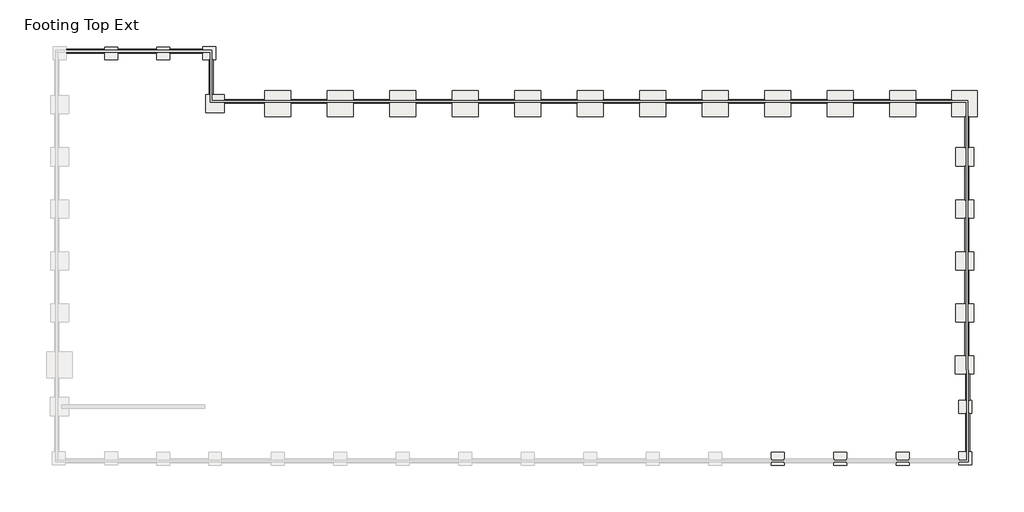
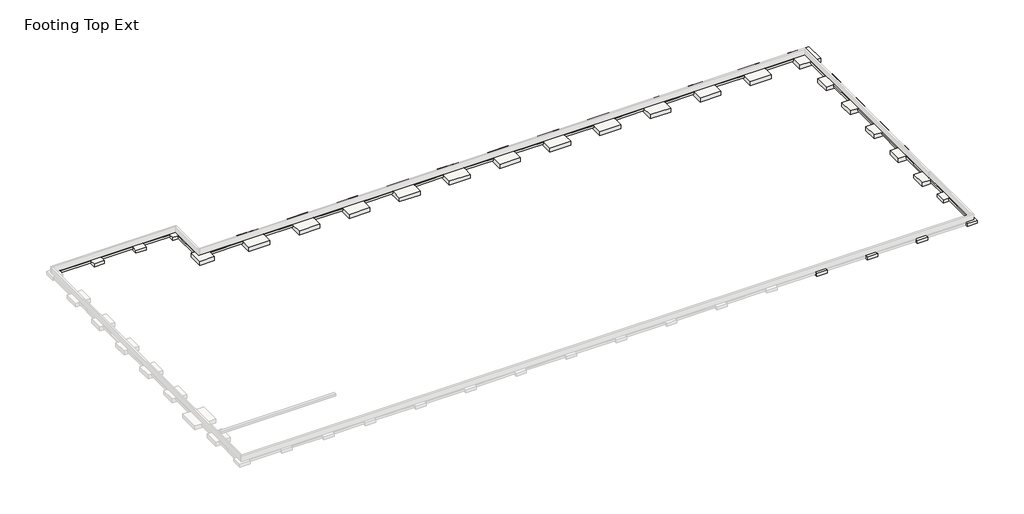
# One storey, part 2 of 2: 26 slabs, 5 footings.
"""IFC4 building model written with IfcOpenShell, lengths in millimetres."""

from ifc_helpers import new_model, si_unit, frame, origin, place, context, project, spatial, polyline, outline, extrude, faceted_brep, element, save

model = new_model("IFC4")

# Units and contexts
model_context = context("Model", 3, world=origin())
ifc_project = project(units=[si_unit("LENGTHUNIT", "METRE", prefix="MILLI")], contexts=[model_context])

# Site, building, storey
site = spatial("IfcSite", under=ifc_project)
building = spatial("IfcBuilding", under=site)
storey = spatial("IfcBuildingStorey", under=building, Name="Footing Top Ext", Elevation=-914.4)

# Footings
placement = place(None, origin())
element("IfcFooting", 1, ObjectType="Bearing Footing - 18\" x 12\"", at=placement, inside=storey, context=model_context, shape_type="SweptSolid", body=[
    extrude(outline(polyline([(305697.0398264, -530975.6413841), (305697.0398264, -530518.4413841), (310230.9398264, -530518.4413841), (310230.9398264, -530975.6413841), (305697.0398264, -530975.6413841)])), frame((0.0, 0.0, -1219.2), z_axis=(0.0, 0.0, 1.0), x_axis=(1.0, 0.0, 0.0)), (0.0, 0.0, 1.0), 304.8),
    extrude(outline(polyline([(317882.6898264, -530975.6413841), (317882.6898264, -530518.4413841), (321806.9898264, -530518.4413841), (321806.9898264, -530975.6413841), (317882.6898264, -530975.6413841)])), frame((0.0, 0.0, -1219.2), z_axis=(0.0, 0.0, 1.0), x_axis=(1.0, 0.0, 0.0)), (0.0, 0.0, 1.0), 304.8),
    extrude(outline(polyline([(316358.6898264, -530518.4413841), (316358.6898264, -530975.6413841), (311754.9398264, -530975.6413841), (311754.9398264, -530518.4413841), (316358.6898264, -530518.4413841)])), frame((0.0, 0.0, -1219.2), z_axis=(0.0, 0.0, 1.0), x_axis=(1.0, 0.0, 0.0)), (0.0, 0.0, 1.0), 304.8),
])
element("IfcFooting", 2, ObjectType="Bearing Footing - 18\" x 12\"", at=placement, inside=storey, context=model_context, shape_type="SweptSolid", body=[
    extrude(outline(polyline([(322537.2398264, -531712.2413841), (322994.4398264, -531712.2413841), (322994.4398264, -535839.7413841), (322537.2398264, -535839.7413841), (322537.2398264, -531712.2413841)])), frame((0.0, 0.0, -1219.2), z_axis=(0.0, 0.0, 1.0), x_axis=(1.0, 0.0, 0.0)), (0.0, 0.0, 1.0), 304.8),
])
element("IfcFooting", 3, ObjectType="Bearing Footing - 18\" x 12\"", at=placement, inside=storey, context=model_context, shape_type="SweptSolid", body=[
    extrude(outline(polyline([(409862.4397781, -536430.2913841), (409862.4397781, -536887.4913841), (405658.7398264, -536887.4913841), (405658.7398264, -536430.2913841), (409862.4397781, -536430.2913841)])), frame((0.0, 0.0, -1219.2), z_axis=(0.0, 0.0, 1.0), x_axis=(1.0, 0.0, 0.0)), (0.0, 0.0, 1.0), 304.8),
    extrude(outline(polyline([(402610.7398264, -536430.2913841), (402610.7398264, -536887.4913841), (398305.4398264, -536887.4913841), (398305.4398264, -536430.2913841), (402610.7398264, -536430.2913841)])), frame((0.0, 0.0, -1219.2), z_axis=(0.0, 0.0, 1.0), x_axis=(1.0, 0.0, 0.0)), (0.0, 0.0, 1.0), 304.8),
    extrude(outline(polyline([(395257.4398264, -536430.2913841), (395257.4398264, -536887.4913841), (390952.1398264, -536887.4913841), (390952.1398264, -536430.2913841), (395257.4398264, -536430.2913841)])), frame((0.0, 0.0, -1219.2), z_axis=(0.0, 0.0, 1.0), x_axis=(1.0, 0.0, 0.0)), (0.0, 0.0, 1.0), 304.8),
    extrude(outline(polyline([(387904.1398264, -536430.2913841), (387904.1398264, -536887.4913841), (383598.8398264, -536887.4913841), (383598.8398264, -536430.2913841), (387904.1398264, -536430.2913841)])), frame((0.0, 0.0, -1219.2), z_axis=(0.0, 0.0, 1.0), x_axis=(1.0, 0.0, 0.0)), (0.0, 0.0, 1.0), 304.8),
    extrude(outline(polyline([(380550.8398264, -536430.2913841), (380550.8398264, -536887.4913841), (376245.5398264, -536887.4913841), (376245.5398264, -536430.2913841), (380550.8398264, -536430.2913841)])), frame((0.0, 0.0, -1219.2), z_axis=(0.0, 0.0, 1.0), x_axis=(1.0, 0.0, 0.0)), (0.0, 0.0, 1.0), 304.8),
    extrude(outline(polyline([(373197.5398264, -536430.2913841), (373197.5398264, -536887.4913841), (368892.2398264, -536887.4913841), (368892.2398264, -536430.2913841), (373197.5398264, -536430.2913841)])), frame((0.0, 0.0, -1219.2), z_axis=(0.0, 0.0, 1.0), x_axis=(1.0, 0.0, 0.0)), (0.0, 0.0, 1.0), 304.8),
    extrude(outline(polyline([(365844.2398264, -536430.2913841), (365844.2398264, -536887.4913841), (361538.9398264, -536887.4913841), (361538.9398264, -536430.2913841), (365844.2398264, -536430.2913841)])), frame((0.0, 0.0, -1219.2), z_axis=(0.0, 0.0, 1.0), x_axis=(1.0, 0.0, 0.0)), (0.0, 0.0, 1.0), 304.8),
    extrude(outline(polyline([(358490.9398264, -536430.2913841), (358490.9398264, -536887.4913841), (354185.6398264, -536887.4913841), (354185.6398264, -536430.2913841), (358490.9398264, -536430.2913841)])), frame((0.0, 0.0, -1219.2), z_axis=(0.0, 0.0, 1.0), x_axis=(1.0, 0.0, 0.0)), (0.0, 0.0, 1.0), 304.8),
    extrude(outline(polyline([(351137.6398264, -536430.2913841), (351137.6398264, -536887.4913841), (346832.3398264, -536887.4913841), (346832.3398264, -536430.2913841), (351137.6398264, -536430.2913841)])), frame((0.0, 0.0, -1219.2), z_axis=(0.0, 0.0, 1.0), x_axis=(1.0, 0.0, 0.0)), (0.0, 0.0, 1.0), 304.8),
    extrude(outline(polyline([(343784.3398264, -536430.2913841), (343784.3398264, -536887.4913841), (339479.0398264, -536887.4913841), (339479.0398264, -536430.2913841), (343784.3398264, -536430.2913841)])), frame((0.0, 0.0, -1219.2), z_axis=(0.0, 0.0, 1.0), x_axis=(1.0, 0.0, 0.0)), (0.0, 0.0, 1.0), 304.8),
    extrude(outline(polyline([(336431.0398264, -536430.2913841), (336431.0398264, -536887.4913841), (332125.7398264, -536887.4913841), (332125.7398264, -536430.2913841), (336431.0398264, -536430.2913841)])), frame((0.0, 0.0, -1219.2), z_axis=(0.0, 0.0, 1.0), x_axis=(1.0, 0.0, 0.0)), (0.0, 0.0, 1.0), 304.8),
    extrude(outline(polyline([(329077.7398264, -536430.2913841), (329077.7398264, -536887.4913841), (324289.8398264, -536887.4913841), (324289.8398264, -536430.2913841), (329077.7398264, -536430.2913841)])), frame((0.0, 0.0, -1219.2), z_axis=(0.0, 0.0, 1.0), x_axis=(1.0, 0.0, 0.0)), (0.0, 0.0, 1.0), 304.8),
])
element("IfcFooting", 4, ObjectType="Bearing Footing - 18\" x 12\"", at=placement, inside=storey, context=model_context, shape_type="SweptSolid", body=[
    extrude(outline(polyline([(411894.4398264, -560496.7913841), (411437.2398264, -560496.7913841), (411437.2398264, -556502.6413841), (411894.4398264, -556502.6413841), (411894.4398264, -560496.7913841)])), frame((0.0, 0.0, -1219.2), z_axis=(0.0, 0.0, 1.0), x_axis=(1.0, 0.0, 0.0)), (0.0, 0.0, 1.0), 304.8),
    extrude(outline(polyline([(411437.2398264, -562630.3913841), (411894.4398264, -562630.3913841), (411894.4398264, -566599.1414082), (411437.2398264, -566599.1414082), (411437.2398264, -562630.3913841)])), frame((0.0, 0.0, -1219.2), z_axis=(0.0, 0.0, 1.0), x_axis=(1.0, 0.0, 0.0)), (0.0, 0.0, 1.0), 304.8),
    extrude(outline(polyline([(411894.4398264, -554369.0413841), (411437.2398264, -554369.0413841), (411437.2398264, -550374.8913841), (411894.4398264, -550374.8913841), (411894.4398264, -554369.0413841)])), frame((0.0, 0.0, -1219.2), z_axis=(0.0, 0.0, 1.0), x_axis=(1.0, 0.0, 0.0)), (0.0, 0.0, 1.0), 304.8),
    extrude(outline(polyline([(411894.4398264, -548241.2913841), (411437.2398264, -548241.2913841), (411437.2398264, -544247.1413841), (411894.4398264, -544247.1413841), (411894.4398264, -548241.2913841)])), frame((0.0, 0.0, -1219.2), z_axis=(0.0, 0.0, 1.0), x_axis=(1.0, 0.0, 0.0)), (0.0, 0.0, 1.0), 304.8),
    extrude(outline(polyline([(411894.4398264, -542113.5413841), (411437.2398264, -542113.5413841), (411437.2398264, -538424.1913358), (411894.4398264, -538424.1913358), (411894.4398264, -542113.5413841)])), frame((0.0, 0.0, -1219.2), z_axis=(0.0, 0.0, 1.0), x_axis=(1.0, 0.0, 0.0)), (0.0, 0.0, 1.0), 304.8),
])
element("IfcFooting", 5, ObjectType="Bearing Footing - 18\" x 12\"", at=placement, inside=storey, context=model_context, shape_type="SweptSolid", body=[
    extrude(outline(polyline([(411983.3398264, -571831.5413841), (411526.1398264, -571831.5413841), (411526.1398264, -568732.7414082), (411983.3398264, -568732.7414082), (411983.3398264, -571831.5413841)])), frame((0.0, 0.0, -1219.2), z_axis=(0.0, 0.0, 1.0), x_axis=(1.0, 0.0, 0.0)), (0.0, 0.0, 1.0), 304.8),
    extrude(outline(polyline([(411526.1398264, -573355.5413841), (411983.3398264, -573355.5413841), (411983.3398264, -577927.5413841), (411526.1398264, -577927.5413841), (411526.1398264, -573355.5413841)])), frame((0.0, 0.0, -1219.2), z_axis=(0.0, 0.0, 1.0), x_axis=(1.0, 0.0, 0.0)), (0.0, 0.0, 1.0), 304.8),
])

# Slabs
element("IfcSlab", 6, ObjectType="Footing-Rectangular : F10", at=placement, inside=storey, context=model_context, shape_type="Brep", body=[
    faceted_brep([(409862.4397781, -535376.1913358, -914.4), (409862.4397781, -536430.2913841, -914.4), (409862.4397781, -536887.4913841, -914.4), (409862.4397781, -538424.1913358, -914.4), (411437.2398264, -538424.1913358, -914.4), (411894.4398264, -538424.1913358, -914.4), (412910.4397781, -538424.1913358, -914.4), (412910.4397781, -535376.1913358, -914.4), (409862.4397781, -535376.1913358, -1524.0), (412910.4397781, -535376.1913358, -1524.0), (412910.4397781, -538424.1913358, -1524.0), (409862.4397781, -538424.1913358, -1524.0)], [[[0, 1, 2, 3, 4, 5, 6, 7]], [[8, 9, 10, 11]], [[3, 2, 1, 0, 8, 11]], [[6, 5, 4, 3, 11, 10]], [[7, 6, 10, 9]], [[0, 7, 9, 8]]]),
])
element("IfcSlab", 7, ObjectType="Footing-Rectangular : F10", at=placement, inside=storey, context=model_context, shape_type="Brep", body=[
    faceted_brep([(402610.7398264, -535382.5413358, -914.4), (402610.7398264, -536430.2913841, -914.4), (402610.7398264, -536887.4913841, -914.4), (402610.7398264, -538430.5413358, -914.4), (405658.7398264, -538430.5413358, -914.4), (405658.7398264, -536887.4913841, -914.4), (405658.7398264, -536430.2913841, -914.4), (405658.7398264, -535382.5413358, -914.4), (402610.7398264, -535382.5413358, -1524.0), (405658.7398264, -535382.5413358, -1524.0), (405658.7398264, -538430.5413358, -1524.0), (402610.7398264, -538430.5413358, -1524.0)], [[[0, 1, 2, 3, 4, 5, 6, 7]], [[8, 9, 10, 11]], [[3, 2, 1, 0, 8, 11]], [[4, 3, 11, 10]], [[7, 6, 5, 4, 10, 9]], [[0, 7, 9, 8]]]),
])
element("IfcSlab", 8, ObjectType="Footing-Rectangular : F10", at=placement, inside=storey, context=model_context, shape_type="Brep", body=[
    faceted_brep([(395257.4398264, -535382.5413358, -914.4), (395257.4398264, -536430.2913841, -914.4), (395257.4398264, -536887.4913841, -914.4), (395257.4398264, -538430.5413358, -914.4), (398305.4398264, -538430.5413358, -914.4), (398305.4398264, -536887.4913841, -914.4), (398305.4398264, -536430.2913841, -914.4), (398305.4398264, -535382.5413358, -914.4), (395257.4398264, -535382.5413358, -1524.0), (398305.4398264, -535382.5413358, -1524.0), (398305.4398264, -538430.5413358, -1524.0), (395257.4398264, -538430.5413358, -1524.0)], [[[0, 1, 2, 3, 4, 5, 6, 7]], [[8, 9, 10, 11]], [[3, 2, 1, 0, 8, 11]], [[4, 3, 11, 10]], [[7, 6, 5, 4, 10, 9]], [[0, 7, 9, 8]]]),
])
element("IfcSlab", 9, ObjectType="Footing-Rectangular : F10", at=placement, inside=storey, context=model_context, shape_type="Brep", body=[
    faceted_brep([(387904.1398264, -535382.5413358, -914.4), (387904.1398264, -536430.2913841, -914.4), (387904.1398264, -536887.4913841, -914.4), (387904.1398264, -538430.5413358, -914.4), (390952.1398264, -538430.5413358, -914.4), (390952.1398264, -536887.4913841, -914.4), (390952.1398264, -536430.2913841, -914.4), (390952.1398264, -535382.5413358, -914.4), (387904.1398264, -535382.5413358, -1524.0), (390952.1398264, -535382.5413358, -1524.0), (390952.1398264, -538430.5413358, -1524.0), (387904.1398264, -538430.5413358, -1524.0)], [[[0, 1, 2, 3, 4, 5, 6, 7]], [[8, 9, 10, 11]], [[3, 2, 1, 0, 8, 11]], [[4, 3, 11, 10]], [[7, 6, 5, 4, 10, 9]], [[0, 7, 9, 8]]]),
])
element("IfcSlab", 10, ObjectType="Footing-Rectangular : F10", at=placement, inside=storey, context=model_context, shape_type="Brep", body=[
    faceted_brep([(380550.8398264, -535382.5413358, -914.4), (380550.8398264, -536430.2913841, -914.4), (380550.8398264, -536887.4913841, -914.4), (380550.8398264, -538430.5413358, -914.4), (383598.8398264, -538430.5413358, -914.4), (383598.8398264, -536887.4913841, -914.4), (383598.8398264, -536430.2913841, -914.4), (383598.8398264, -535382.5413358, -914.4), (380550.8398264, -535382.5413358, -1524.0), (383598.8398264, -535382.5413358, -1524.0), (383598.8398264, -538430.5413358, -1524.0), (380550.8398264, -538430.5413358, -1524.0)], [[[0, 1, 2, 3, 4, 5, 6, 7]], [[8, 9, 10, 11]], [[3, 2, 1, 0, 8, 11]], [[4, 3, 11, 10]], [[7, 6, 5, 4, 10, 9]], [[0, 7, 9, 8]]]),
])
element("IfcSlab", 11, ObjectType="Footing-Rectangular : F10", at=placement, inside=storey, context=model_context, shape_type="Brep", body=[
    faceted_brep([(373197.5398264, -535382.5413358, -914.4), (373197.5398264, -536430.2913841, -914.4), (373197.5398264, -536887.4913841, -914.4), (373197.5398264, -538430.5413358, -914.4), (376245.5398264, -538430.5413358, -914.4), (376245.5398264, -536887.4913841, -914.4), (376245.5398264, -536430.2913841, -914.4), (376245.5398264, -535382.5413358, -914.4), (373197.5398264, -535382.5413358, -1524.0), (376245.5398264, -535382.5413358, -1524.0), (376245.5398264, -538430.5413358, -1524.0), (373197.5398264, -538430.5413358, -1524.0)], [[[0, 1, 2, 3, 4, 5, 6, 7]], [[8, 9, 10, 11]], [[3, 2, 1, 0, 8, 11]], [[4, 3, 11, 10]], [[7, 6, 5, 4, 10, 9]], [[0, 7, 9, 8]]]),
])
element("IfcSlab", 12, ObjectType="Footing-Rectangular : F10", at=placement, inside=storey, context=model_context, shape_type="Brep", body=[
    faceted_brep([(365844.2398264, -535382.5413358, -914.4), (365844.2398264, -536430.2913841, -914.4), (365844.2398264, -536887.4913841, -914.4), (365844.2398264, -538430.5413358, -914.4), (368892.2398264, -538430.5413358, -914.4), (368892.2398264, -536887.4913841, -914.4), (368892.2398264, -536430.2913841, -914.4), (368892.2398264, -535382.5413358, -914.4), (365844.2398264, -535382.5413358, -1524.0), (368892.2398264, -535382.5413358, -1524.0), (368892.2398264, -538430.5413358, -1524.0), (365844.2398264, -538430.5413358, -1524.0)], [[[0, 1, 2, 3, 4, 5, 6, 7]], [[8, 9, 10, 11]], [[3, 2, 1, 0, 8, 11]], [[4, 3, 11, 10]], [[7, 6, 5, 4, 10, 9]], [[0, 7, 9, 8]]]),
])
element("IfcSlab", 13, ObjectType="Footing-Rectangular : F10", at=placement, inside=storey, context=model_context, shape_type="Brep", body=[
    faceted_brep([(358490.9398264, -535382.5413358, -914.4), (358490.9398264, -536430.2913841, -914.4), (358490.9398264, -536887.4913841, -914.4), (358490.9398264, -538430.5413358, -914.4), (361538.9398264, -538430.5413358, -914.4), (361538.9398264, -536887.4913841, -914.4), (361538.9398264, -536430.2913841, -914.4), (361538.9398264, -535382.5413358, -914.4), (358490.9398264, -535382.5413358, -1524.0), (361538.9398264, -535382.5413358, -1524.0), (361538.9398264, -538430.5413358, -1524.0), (358490.9398264, -538430.5413358, -1524.0)], [[[0, 1, 2, 3, 4, 5, 6, 7]], [[8, 9, 10, 11]], [[3, 2, 1, 0, 8, 11]], [[4, 3, 11, 10]], [[7, 6, 5, 4, 10, 9]], [[0, 7, 9, 8]]]),
])
element("IfcSlab", 14, ObjectType="Footing-Rectangular : F10", at=placement, inside=storey, context=model_context, shape_type="Brep", body=[
    faceted_brep([(351137.6398264, -535382.5413358, -914.4), (351137.6398264, -536430.2913841, -914.4), (351137.6398264, -536887.4913841, -914.4), (351137.6398264, -538430.5413358, -914.4), (354185.6398264, -538430.5413358, -914.4), (354185.6398264, -536887.4913841, -914.4), (354185.6398264, -536430.2913841, -914.4), (354185.6398264, -535382.5413358, -914.4), (351137.6398264, -535382.5413358, -1524.0), (354185.6398264, -535382.5413358, -1524.0), (354185.6398264, -538430.5413358, -1524.0), (351137.6398264, -538430.5413358, -1524.0)], [[[0, 1, 2, 3, 4, 5, 6, 7]], [[8, 9, 10, 11]], [[3, 2, 1, 0, 8, 11]], [[4, 3, 11, 10]], [[7, 6, 5, 4, 10, 9]], [[0, 7, 9, 8]]]),
])
element("IfcSlab", 15, ObjectType="Footing-Rectangular : F10", at=placement, inside=storey, context=model_context, shape_type="Brep", body=[
    faceted_brep([(343784.3398264, -535382.5413358, -914.4), (343784.3398264, -536430.2913841, -914.4), (343784.3398264, -536887.4913841, -914.4), (343784.3398264, -538430.5413358, -914.4), (346832.3398264, -538430.5413358, -914.4), (346832.3398264, -536887.4913841, -914.4), (346832.3398264, -536430.2913841, -914.4), (346832.3398264, -535382.5413358, -914.4), (343784.3398264, -535382.5413358, -1524.0), (346832.3398264, -535382.5413358, -1524.0), (346832.3398264, -538430.5413358, -1524.0), (343784.3398264, -538430.5413358, -1524.0)], [[[0, 1, 2, 3, 4, 5, 6, 7]], [[8, 9, 10, 11]], [[3, 2, 1, 0, 8, 11]], [[4, 3, 11, 10]], [[7, 6, 5, 4, 10, 9]], [[0, 7, 9, 8]]]),
])
element("IfcSlab", 16, ObjectType="Footing-Rectangular : F10", at=placement, inside=storey, context=model_context, shape_type="Brep", body=[
    faceted_brep([(336431.0398264, -535382.5413358, -914.4), (336431.0398264, -536430.2913841, -914.4), (336431.0398264, -536887.4913841, -914.4), (336431.0398264, -538430.5413358, -914.4), (339479.0398264, -538430.5413358, -914.4), (339479.0398264, -536887.4913841, -914.4), (339479.0398264, -536430.2913841, -914.4), (339479.0398264, -535382.5413358, -914.4), (336431.0398264, -535382.5413358, -1524.0), (339479.0398264, -535382.5413358, -1524.0), (339479.0398264, -538430.5413358, -1524.0), (336431.0398264, -538430.5413358, -1524.0)], [[[0, 1, 2, 3, 4, 5, 6, 7]], [[8, 9, 10, 11]], [[3, 2, 1, 0, 8, 11]], [[4, 3, 11, 10]], [[7, 6, 5, 4, 10, 9]], [[0, 7, 9, 8]]]),
])
element("IfcSlab", 17, ObjectType="Footing-Rectangular : F10", at=placement, inside=storey, context=model_context, shape_type="Brep", body=[
    faceted_brep([(329077.7398264, -535382.5413358, -914.4), (329077.7398264, -536430.2913841, -914.4), (329077.7398264, -536887.4913841, -914.4), (329077.7398264, -538430.5413358, -914.4), (332125.7398264, -538430.5413358, -914.4), (332125.7398264, -536887.4913841, -914.4), (332125.7398264, -536430.2913841, -914.4), (332125.7398264, -535382.5413358, -914.4), (329077.7398264, -535382.5413358, -1524.0), (332125.7398264, -535382.5413358, -1524.0), (332125.7398264, -538430.5413358, -1524.0), (329077.7398264, -538430.5413358, -1524.0)], [[[0, 1, 2, 3, 4, 5, 6, 7]], [[8, 9, 10, 11]], [[3, 2, 1, 0, 8, 11]], [[4, 3, 11, 10]], [[7, 6, 5, 4, 10, 9]], [[0, 7, 9, 8]]]),
])
element("IfcSlab", 18, ObjectType="Footing-Rectangular : F5", at=placement, inside=storey, context=model_context, shape_type="Brep", body=[
    faceted_brep([(317882.6898264, -530245.3913841, -914.4), (316358.6898264, -530245.3913841, -914.4), (316358.6898264, -530518.4413841, -914.4), (316358.6898264, -530975.6413841, -914.4), (316358.6898264, -531769.3913841, -914.4), (317882.6898264, -531769.3913841, -914.4), (317882.6898264, -530975.6413841, -914.4), (317882.6898264, -530518.4413841, -914.4), (317882.6898264, -530245.3913841, -1371.6), (317882.6898264, -531769.3913841, -1371.6), (316358.6898264, -531769.3913841, -1371.6), (316358.6898264, -530245.3913841, -1371.6)], [[[0, 1, 2, 3, 4, 5, 6, 7]], [[8, 9, 10, 11]], [[1, 0, 8, 11]], [[4, 3, 2, 1, 11, 10]], [[5, 4, 10, 9]], [[0, 7, 6, 5, 9, 8]]]),
])
element("IfcSlab", 19, ObjectType="Footing-Rectangular : F5", at=placement, inside=storey, context=model_context, shape_type="Brep", body=[
    faceted_brep([(311754.9398264, -530245.3913841, -914.4), (310230.9398264, -530245.3913841, -914.4), (310230.9398264, -530518.4413841, -914.4), (310230.9398264, -530975.6413841, -914.4), (310230.9398264, -531769.3913841, -914.4), (311754.9398264, -531769.3913841, -914.4), (311754.9398264, -530975.6413841, -914.4), (311754.9398264, -530518.4413841, -914.4), (311754.9398264, -530245.3913841, -1371.6), (311754.9398264, -531769.3913841, -1371.6), (310230.9398264, -531769.3913841, -1371.6), (310230.9398264, -530245.3913841, -1371.6)], [[[0, 1, 2, 3, 4, 5, 6, 7]], [[8, 9, 10, 11]], [[1, 0, 8, 11]], [[4, 3, 2, 1, 11, 10]], [[5, 4, 10, 9]], [[0, 7, 6, 5, 9, 8]]]),
])
element("IfcSlab", 20, ObjectType="Footing-Rectangular : F5", at=placement, inside=storey, context=model_context, shape_type="Brep", body=[
    faceted_brep([(323330.9898264, -530188.2413841, -914.4), (321806.9898264, -530188.2413841, -914.4), (321806.9898264, -530518.4413841, -914.4), (321806.9898264, -530975.6413841, -914.4), (321806.9898264, -531712.2413841, -914.4), (322537.2398264, -531712.2413841, -914.4), (322994.4398264, -531712.2413841, -914.4), (323330.9898264, -531712.2413841, -914.4), (323330.9898264, -530188.2413841, -1371.6), (323330.9898264, -531712.2413841, -1371.6), (321806.9898264, -531712.2413841, -1371.6), (321806.9898264, -530188.2413841, -1371.6)], [[[0, 1, 2, 3, 4, 5, 6, 7]], [[8, 9, 10, 11]], [[1, 0, 8, 11]], [[4, 3, 2, 1, 11, 10]], [[7, 6, 5, 4, 10, 9]], [[0, 7, 9, 8]]]),
])
element("IfcSlab", 21, ObjectType="Footing-Rectangular : F5", at=placement, inside=storey, context=model_context, shape_type="Brep", body=[
    faceted_brep([(390190.1398264, -577978.3413841, -914.4), (388666.1398264, -577978.3413841, -914.4), (388666.1398264, -578759.3913841, -914.4), (388666.1398264, -579216.5913841, -914.4), (388666.1398264, -579502.3413841, -914.4), (390190.1398264, -579502.3413841, -914.4), (390190.1398264, -579216.5913841, -914.4), (390190.1398264, -578759.3913841, -914.4), (390190.1398264, -577978.3413841, -1371.6), (390190.1398264, -579502.3413841, -1371.6), (388666.1398264, -579502.3413841, -1371.6), (388666.1398264, -577978.3413841, -1371.6)], [[[0, 1, 2, 3, 4, 5, 6, 7]], [[8, 9, 10, 11]], [[1, 0, 8, 11]], [[4, 3, 2, 1, 11, 10]], [[5, 4, 10, 9]], [[0, 7, 6, 5, 9, 8]]]),
])
element("IfcSlab", 22, ObjectType="Footing-Rectangular : F5", at=placement, inside=storey, context=model_context, shape_type="Brep", body=[
    faceted_brep([(397543.4398264, -577971.9913841, -914.4), (396019.4398264, -577971.9913841, -914.4), (396019.4398264, -578759.3913841, -914.4), (396019.4398264, -579216.5913841, -914.4), (396019.4398264, -579495.9913841, -914.4), (397543.4398264, -579495.9913841, -914.4), (397543.4398264, -579216.5913841, -914.4), (397543.4398264, -578759.3913841, -914.4), (397543.4398264, -577971.9913841, -1371.6), (397543.4398264, -579495.9913841, -1371.6), (396019.4398264, -579495.9913841, -1371.6), (396019.4398264, -577971.9913841, -1371.6)], [[[0, 1, 2, 3, 4, 5, 6, 7]], [[8, 9, 10, 11]], [[1, 0, 8, 11]], [[4, 3, 2, 1, 11, 10]], [[5, 4, 10, 9]], [[0, 7, 6, 5, 9, 8]]]),
])
element("IfcSlab", 23, ObjectType="Footing-Rectangular : F5", at=placement, inside=storey, context=model_context, shape_type="Brep", body=[
    faceted_brep([(404896.7398264, -577971.9913841, -914.4), (403372.7398264, -577971.9913841, -914.4), (403372.7398264, -578759.3913841, -914.4), (403372.7398264, -579216.5913841, -914.4), (403372.7398264, -579495.9913841, -914.4), (404896.7398264, -579495.9913841, -914.4), (404896.7398264, -579216.5913841, -914.4), (404896.7398264, -578759.3913841, -914.4), (404896.7398264, -577971.9913841, -1371.6), (404896.7398264, -579495.9913841, -1371.6), (403372.7398264, -579495.9913841, -1371.6), (403372.7398264, -577971.9913841, -1371.6)], [[[0, 1, 2, 3, 4, 5, 6, 7]], [[8, 9, 10, 11]], [[1, 0, 8, 11]], [[4, 3, 2, 1, 11, 10]], [[5, 4, 10, 9]], [[0, 7, 6, 5, 9, 8]]]),
])
element("IfcSlab", 24, ObjectType="Footing-Rectangular : F5", at=placement, inside=storey, context=model_context, shape_type="Brep", body=[
    faceted_brep([(412218.2898264, -571831.5413841, -914.4), (411983.3398264, -571831.5413841, -914.4), (411526.1398264, -571831.5413841, -914.4), (410694.2898264, -571831.5413841, -914.4), (410694.2898264, -573355.5413841, -914.4), (411526.1398264, -573355.5413841, -914.4), (411983.3398264, -573355.5413841, -914.4), (412218.2898264, -573355.5413841, -914.4), (412218.2898264, -571831.5413841, -1371.6), (412218.2898264, -573355.5413841, -1371.6), (410694.2898264, -573355.5413841, -1371.6), (410694.2898264, -571831.5413841, -1371.6)], [[[0, 1, 2, 3, 4, 5, 6, 7]], [[8, 9, 10, 11]], [[3, 2, 1, 0, 8, 11]], [[4, 3, 11, 10]], [[7, 6, 5, 4, 10, 9]], [[0, 7, 9, 8]]]),
])
element("IfcSlab", 25, ObjectType="Footing-Rectangular : F5", at=placement, inside=storey, context=model_context, shape_type="Brep", body=[
    faceted_brep([(412224.6398264, -577927.5413841, -914.4), (411983.3398264, -577927.5413841, -914.4), (411526.1398264, -577927.5413841, -914.4), (410700.6398264, -577927.5413841, -914.4), (410700.6398264, -578759.3913841, -914.4), (410700.6398264, -579216.5913841, -914.4), (410700.6398264, -579451.5413841, -914.4), (412224.6398264, -579451.5413841, -914.4), (412224.6398264, -577927.5413841, -1371.6), (412224.6398264, -579451.5413841, -1371.6), (410700.6398264, -579451.5413841, -1371.6), (410700.6398264, -577927.5413841, -1371.6)], [[[0, 1, 2, 3, 4, 5, 6, 7]], [[8, 9, 10, 11]], [[3, 2, 1, 0, 8, 11]], [[6, 5, 4, 3, 11, 10]], [[7, 6, 10, 9]], [[0, 7, 9, 8]]]),
])
element("IfcSlab", 26, ObjectType="Footing-Rectangular : F7", at=placement, inside=storey, context=model_context, shape_type="Brep", body=[
    faceted_brep([(410319.6398264, -566599.1414082, -914.4), (410319.6398264, -568732.7414082, -914.4), (411526.1398264, -568732.7414082, -914.4), (411983.3398264, -568732.7414082, -914.4), (412453.2398264, -568732.7414082, -914.4), (412453.2398264, -566599.1414082, -914.4), (411894.4398264, -566599.1414082, -914.4), (411437.2398264, -566599.1414082, -914.4), (410319.6398264, -566599.1414082, -1524.0), (412453.2398264, -566599.1414082, -1524.0), (412453.2398264, -568732.7414082, -1524.0), (410319.6398264, -568732.7414082, -1524.0)], [[[0, 1, 2, 3, 4, 5, 6, 7]], [[8, 9, 10, 11]], [[1, 0, 8, 11]], [[4, 3, 2, 1, 11, 10]], [[5, 4, 10, 9]], [[0, 7, 6, 5, 9, 8]]]),
])
element("IfcSlab", 27, ObjectType="Footing-Rectangular : F7", at=placement, inside=storey, context=model_context, shape_type="Brep", body=[
    faceted_brep([(412484.9898264, -560496.7913841, -914.4), (411894.4398264, -560496.7913841, -914.4), (411437.2398264, -560496.7913841, -914.4), (410351.3898264, -560496.7913841, -914.4), (410351.3898264, -562630.3913841, -914.4), (411437.2398264, -562630.3913841, -914.4), (411894.4398264, -562630.3913841, -914.4), (412484.9898264, -562630.3913841, -914.4), (412484.9898264, -560496.7913841, -1524.0), (412484.9898264, -562630.3913841, -1524.0), (410351.3898264, -562630.3913841, -1524.0), (410351.3898264, -560496.7913841, -1524.0)], [[[0, 1, 2, 3, 4, 5, 6, 7]], [[8, 9, 10, 11]], [[3, 2, 1, 0, 8, 11]], [[4, 3, 11, 10]], [[7, 6, 5, 4, 10, 9]], [[0, 7, 9, 8]]]),
])
element("IfcSlab", 28, ObjectType="Footing-Rectangular : F7", at=placement, inside=storey, context=model_context, shape_type="Brep", body=[
    faceted_brep([(412484.9898264, -554369.0413841, -914.4), (411894.4398264, -554369.0413841, -914.4), (411437.2398264, -554369.0413841, -914.4), (410351.3898264, -554369.0413841, -914.4), (410351.3898264, -556502.6413841, -914.4), (411437.2398264, -556502.6413841, -914.4), (411894.4398264, -556502.6413841, -914.4), (412484.9898264, -556502.6413841, -914.4), (412484.9898264, -554369.0413841, -1524.0), (412484.9898264, -556502.6413841, -1524.0), (410351.3898264, -556502.6413841, -1524.0), (410351.3898264, -554369.0413841, -1524.0)], [[[0, 1, 2, 3, 4, 5, 6, 7]], [[8, 9, 10, 11]], [[3, 2, 1, 0, 8, 11]], [[4, 3, 11, 10]], [[7, 6, 5, 4, 10, 9]], [[0, 7, 9, 8]]]),
])
element("IfcSlab", 29, ObjectType="Footing-Rectangular : F7", at=placement, inside=storey, context=model_context, shape_type="Brep", body=[
    faceted_brep([(412484.9898264, -548241.2913841, -914.4), (411894.4398264, -548241.2913841, -914.4), (411437.2398264, -548241.2913841, -914.4), (410351.3898264, -548241.2913841, -914.4), (410351.3898264, -550374.8913841, -914.4), (411437.2398264, -550374.8913841, -914.4), (411894.4398264, -550374.8913841, -914.4), (412484.9898264, -550374.8913841, -914.4), (412484.9898264, -548241.2913841, -1524.0), (412484.9898264, -550374.8913841, -1524.0), (410351.3898264, -550374.8913841, -1524.0), (410351.3898264, -548241.2913841, -1524.0)], [[[0, 1, 2, 3, 4, 5, 6, 7]], [[8, 9, 10, 11]], [[3, 2, 1, 0, 8, 11]], [[4, 3, 11, 10]], [[7, 6, 5, 4, 10, 9]], [[0, 7, 9, 8]]]),
])
element("IfcSlab", 30, ObjectType="Footing-Rectangular : F7", at=placement, inside=storey, context=model_context, shape_type="Brep", body=[
    faceted_brep([(412478.6398264, -542113.5413841, -914.4), (411894.4398264, -542113.5413841, -914.4), (411437.2398264, -542113.5413841, -914.4), (410345.0398264, -542113.5413841, -914.4), (410345.0398264, -544247.1413841, -914.4), (411437.2398264, -544247.1413841, -914.4), (411894.4398264, -544247.1413841, -914.4), (412478.6398264, -544247.1413841, -914.4), (412478.6398264, -542113.5413841, -1524.0), (412478.6398264, -544247.1413841, -1524.0), (410345.0398264, -544247.1413841, -1524.0), (410345.0398264, -542113.5413841, -1524.0)], [[[0, 1, 2, 3, 4, 5, 6, 7]], [[8, 9, 10, 11]], [[3, 2, 1, 0, 8, 11]], [[4, 3, 11, 10]], [[7, 6, 5, 4, 10, 9]], [[0, 7, 9, 8]]]),
])
element("IfcSlab", 31, ObjectType="Footing-Rectangular : F7", at=placement, inside=storey, context=model_context, shape_type="Brep", body=[
    faceted_brep([(322156.2398264, -535839.7413841, -914.4), (322156.2398264, -537973.3413841, -914.4), (324289.8398264, -537973.3413841, -914.4), (324289.8398264, -536887.4913841, -914.4), (324289.8398264, -536430.2913841, -914.4), (324289.8398264, -535839.7413841, -914.4), (322994.4398264, -535839.7413841, -914.4), (322537.2398264, -535839.7413841, -914.4), (322156.2398264, -535839.7413841, -1524.0), (324289.8398264, -535839.7413841, -1524.0), (324289.8398264, -537973.3413841, -1524.0), (322156.2398264, -537973.3413841, -1524.0)], [[[0, 1, 2, 3, 4, 5, 6, 7]], [[8, 9, 10, 11]], [[1, 0, 8, 11]], [[2, 1, 11, 10]], [[5, 4, 3, 2, 10, 9]], [[0, 7, 6, 5, 9, 8]]]),
])

save(model, "model.ifc")

# Revit data of these elements
# Type "Bearing Footing - 18\" x 12\""
#   Assembly Code = "A1010110"
# Type "Footing-Rectangular : F10"
#   Assembly Code = "A1010100"
#   Width = 10' - 0"
#   Length = 10' - 0"
#   Thickness = 2' - 0"
#   Structural Material [instance default] = CONCRETE FOOTING - SEE STRUCT DWGS.
# Type "Footing-Rectangular : F5"
#   Assembly Code = "A1010100"
#   Width = 5' - 0"
#   Length = 5' - 0"
#   Thickness = 1' - 6"
#   Structural Material [instance default] = CONCRETE FOOTING - SEE STRUCT DWGS.
# Type "Footing-Rectangular : F7"
#   Assembly Code = "A1010100"
#   Width = 7' - 0"
#   Length = 7' - 0"
#   Thickness = 2' - 0"
#   Structural Material [instance default] = CONCRETE FOOTING - SEE STRUCT DWGS.
# Elements 1, 2, 3, 4, 5 (IfcFooting, "Bearing Footing - 18\" x 12\"")
#   Phase Created = New Construction
#   Materials on its faces: "CONCRETE FOOTING - SEE STRUCT DWGS."
# Elements 6, 7, 8, 9, 10, 11, 12, 13, 14, 15, 16, 17 (IfcSlab, "Footing-Rectangular : F10")
#   Comments = ""
#   Structural Material = CONCRETE FOOTING - SEE STRUCT DWGS.
#   Phase Created = New Construction
#   Materials on its faces: "CONCRETE FOOTING - SEE STRUCT DWGS."
# Elements 18, 19, 20, 21, 22, 23, 24, 25 (IfcSlab, "Footing-Rectangular : F5")
#   Comments = ""
#   Structural Material = CONCRETE FOOTING - SEE STRUCT DWGS.
#   Phase Created = New Construction
#   Materials on its faces: "CONCRETE FOOTING - SEE STRUCT DWGS."
# Elements 26, 27, 28, 29, 30, 31 (IfcSlab, "Footing-Rectangular : F7")
#   Comments = ""
#   Structural Material = CONCRETE FOOTING - SEE STRUCT DWGS.
#   Phase Created = New Construction
#   Materials on its faces: "CONCRETE FOOTING - SEE STRUCT DWGS."
# Materials
#   "CONCRETE FOOTING - SEE STRUCT DWGS.": class "Concrete", colour RGB 192 192 192, transparency 0, Description = "Cast-in-place concrete", Cost = 0
